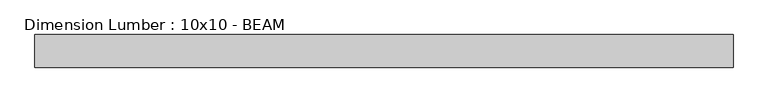
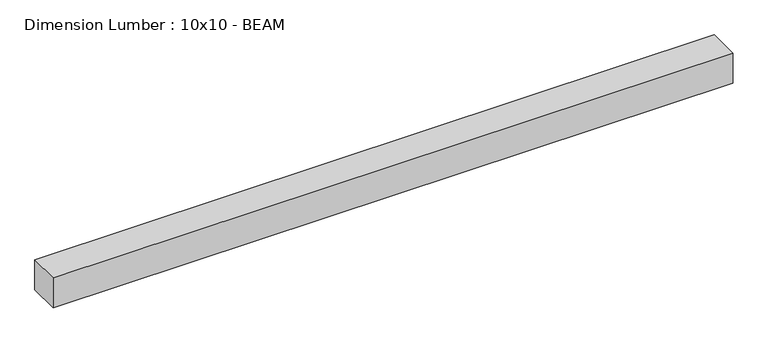
"""IFC4 building model written with IfcOpenShell, lengths in millimetres: beam geometry, Dimension Lumber : 10x10 - BEAM."""

from ifc_helpers import new_model, si_unit, frame, origin, place, context, project, spatial, polyline, outline, extrude, source, transform, mapped, element, save


def dimension_lumber_10x10_beam_f930df24(model_context):
    return source(origin(), model_context, "Body", "SweptSolid", [
        extrude(outline(polyline([(2514.6, 117.475), (2514.6, -117.475), (-2514.6, -117.475), (-2514.6, 117.475), (2514.6, 117.475)])), frame((0.0, 0.0, -117.475), z_axis=(0.0, 0.0, 1.0), x_axis=(1.0, 0.0, 0.0)), (0.0, 0.0, 1.0), 234.95),
    ])


if __name__ == "__main__":
    model = new_model("IFC4")
    model_context = context("Model", 3, world=origin())
    ifc_project = project(units=[si_unit("LENGTHUNIT", "METRE", prefix="MILLI")], contexts=[model_context])
    site = spatial("IfcSite", under=ifc_project)
    building = spatial("IfcBuilding", under=site)
    placement = place(None, origin())
    dimension_lumber_10x10_beam_shape = dimension_lumber_10x10_beam_f930df24(model_context)
    element("IfcBeam", 1, ObjectType="Dimension Lumber : 10x10 - BEAM", at=placement, inside=building, context=model_context, shape_type="MappedRepresentation", body=[
        mapped(dimension_lumber_10x10_beam_shape, transform((0.0, 0.0, 0.0), x_axis=(1.0, 0.0, 0.0), y_axis=(0.0, 1.0, 0.0), z_axis=(0.0, 0.0, 1.0))),
    ])
    save(model, "model.ifc")

# Revit data of these elements
# Type "Dimension Lumber : 10x10 - BEAM"
#   Assembly Code = "B10"
#   A = 0.0755556 SF
#   Length [instance default] = 5' - 0"
#   b = 0' - 9 1/4"
#   d = 0' - 9 1/4"
#   Structural Material = (4) CHARRED SISTERED 2X10s AT BEAM
# Element 1 (IfcBeam, "Dimension Lumber : 10x10 - BEAM")
#   Materials on its faces: "(4) CHARRED SISTERED 2X10s AT BEAM"
# Materials
#   "(4) CHARRED SISTERED 2X10s AT BEAM": class "Wood", colour RGB 144 144 144, transparency 0, Description = "Pinus Echinata", Cost = 0
